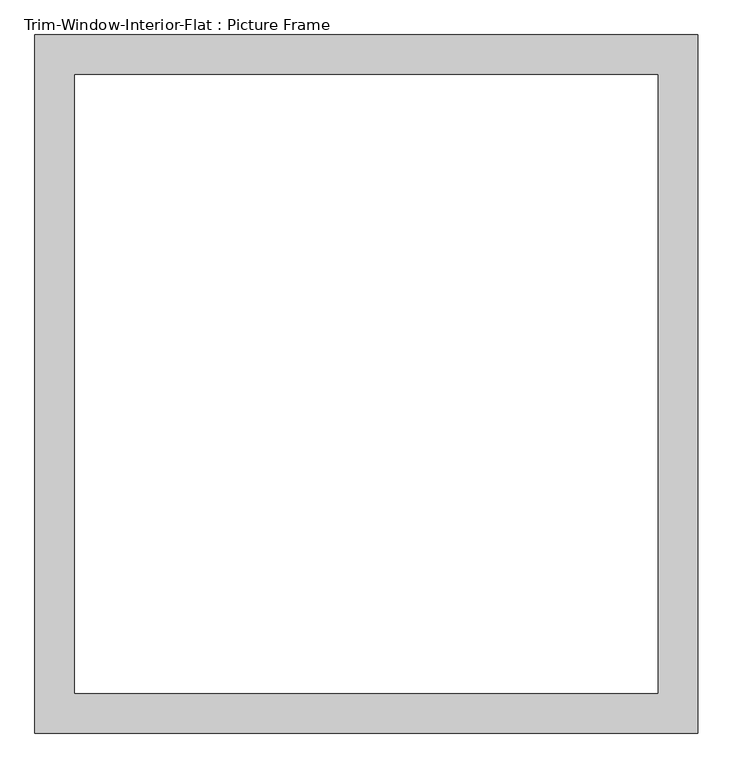
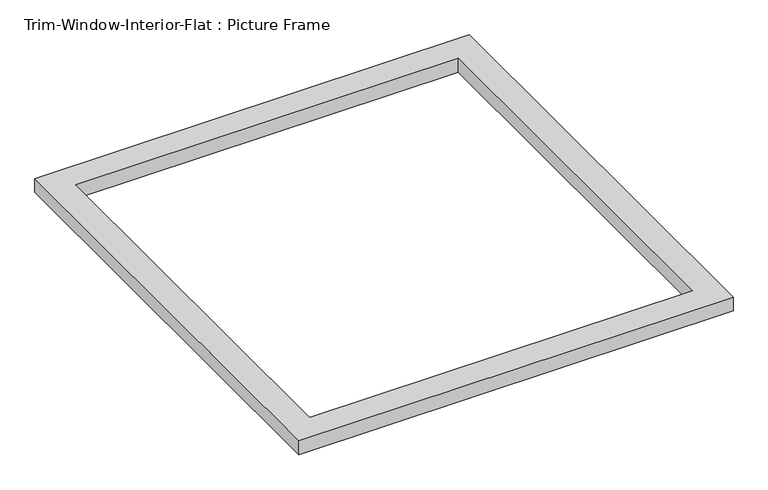
"""IFC4 building model written with IfcOpenShell, lengths in millimetres: proxy geometry, Trim-Window-Interior-Flat : Picture Frame."""

import ifcopenshell
import ifcopenshell.guid

model = None  # the IFC model being written
_history = None  # IfcOwnerHistory: only IFC2X3 demands one
_inside = {}  # id of a spatial element -> (the spatial element, [elements in it])
_under = {}  # id of a project, library or spatial element -> (it, [spatial elements below it])
_declared = {}  # id of a project -> (the project, [libraries it declares])
_typed = {}  # id of a type object -> (the type object, [elements of that type])
_made_of = {}  # id of a material, layer set ... -> (it, [elements and type objects made of it])


def new_model(schema):
    """Start an empty IFC model of exactly this schema.

    Asked for "IFC4X3", IfcOpenShell would pick the latest addendum, in which some entities
    have other attributes; the version numbers below select the first issue.
    IFC2X3 requires an IfcOwnerHistory on every rooted entity: one is made here for all.
    """
    global model, _history
    if schema == "IFC4X3":
        model = ifcopenshell.file(schema_version=(4, 3, 0, 0))
    else:
        model = ifcopenshell.file(schema=schema)
    _inside.clear()
    _under.clear()
    _declared.clear()
    _typed.clear()
    _made_of.clear()
    _history = None
    if model.schema == "IFC2X3":
        org = make("IfcOrganization", Name="unknown")
        user = make(
            "IfcPersonAndOrganization",
            ThePerson=make("IfcPerson", FamilyName="unknown"),
            TheOrganization=org,
        )
        app = make(
            "IfcApplication",
            ApplicationDeveloper=org,
            Version="unknown",
            ApplicationFullName="unknown",
            ApplicationIdentifier="unknown",
        )
        _history = make(
            "IfcOwnerHistory",
            OwningUser=user,
            OwningApplication=app,
            ChangeAction="ADDED",
            CreationDate=0,
        )
    return model


def make(cls, **values):
    """One entity of the class cls with the attributes given. An attribute that is None is left unset."""
    return model.create_entity(
        cls, **{name: value for name, value in values.items() if value is not None}
    )


def rooted(cls, **values):
    """An entity with a GlobalId (a new one), such as an element, a storey or a relation."""
    return make(cls, GlobalId=ifcopenshell.guid.new(), OwnerHistory=_history, **values)


def si_unit(unit_type, name, prefix=None):
    """IfcSIUnit, for example si_unit("LENGTHUNIT", "METRE", prefix="MILLI")."""
    return make("IfcSIUnit", UnitType=unit_type, Prefix=prefix, Name=name)


def assignment(units):
    """IfcUnitAssignment: the units of a project."""
    return None if units is None else make("IfcUnitAssignment", Units=units)


def point(xyz):
    """IfcCartesianPoint."""
    return None if xyz is None else make("IfcCartesianPoint", Coordinates=xyz)


def direction(xyz):
    """IfcDirection."""
    return None if xyz is None else make("IfcDirection", DirectionRatios=xyz)


def frame(location, z_axis=None, x_axis=None):
    """IfcAxis2Placement3D, a coordinate frame: its origin and axes. An axis left out is left unset."""
    return make(
        "IfcAxis2Placement3D",
        Location=point(location),
        Axis=direction(z_axis),
        RefDirection=direction(x_axis),
    )


def origin():
    """The frame at (0, 0, 0) with its axes left unset."""
    return frame((0.0, 0.0, 0.0))


def origin_with_axes():
    """The frame at (0, 0, 0) with the z axis (0, 0, 1) and the x axis (1, 0, 0) written out."""
    return frame((0.0, 0.0, 0.0), z_axis=(0.0, 0.0, 1.0), x_axis=(1.0, 0.0, 0.0))


def place(relative_to, where):
    """IfcLocalPlacement: puts the frame where relative to a parent placement (None: the world)."""
    return make(
        "IfcLocalPlacement", PlacementRelTo=relative_to, RelativePlacement=where
    )


def context(
    kind, dimensions, precision=None, world=None, true_north=None, identifier=None
):
    """IfcGeometricRepresentationContext, for example the 3D "Model" context."""
    return make(
        "IfcGeometricRepresentationContext",
        ContextIdentifier=identifier,
        ContextType=kind,
        CoordinateSpaceDimension=dimensions,
        Precision=precision,
        WorldCoordinateSystem=world,
        TrueNorth=true_north,
    )


def project(units=None, contexts=None):
    """IfcProject with its units and contexts."""
    return rooted(
        "IfcProject",
        Name="project",
        RepresentationContexts=contexts,
        UnitsInContext=assignment(units),
    )


def spatial(cls, under=None, at=None, **own):
    """A site, building, storey or space (cls), placed at a placement, below another one or the project."""
    s = rooted(cls, ObjectPlacement=at, **own)
    if under is not None:
        _under.setdefault(under.id(), (under, []))[1].append(s)
    return s


def polyline(points):
    """IfcPolyline through the points."""
    return make("IfcPolyline", Points=[point(p) for p in points])


def outline(outer, holes=None, kind="AREA"):
    """IfcArbitraryClosedProfileDef: a profile drawn as a closed curve; with holes, ...WithVoids."""
    if holes is None:
        return make("IfcArbitraryClosedProfileDef", ProfileType=kind, OuterCurve=outer)
    return make(
        "IfcArbitraryProfileDefWithVoids",
        ProfileType=kind,
        OuterCurve=outer,
        InnerCurves=holes,
    )


def extrude(swept, where, along, depth):
    """IfcExtrudedAreaSolid: the profile swept, set in the frame where, extruded along a direction by depth."""
    return make(
        "IfcExtrudedAreaSolid",
        SweptArea=swept,
        Position=where,
        ExtrudedDirection=direction(along),
        Depth=depth,
    )


def shape(context_of_items, identifier, shape_type, items):
    """IfcShapeRepresentation: the items that make up one representation, for example the "Body"."""
    return make(
        "IfcShapeRepresentation",
        ContextOfItems=context_of_items,
        RepresentationIdentifier=identifier,
        RepresentationType=shape_type,
        Items=items,
    )


def source(mapping_origin, context_of_items, identifier, shape_type, items):
    """IfcRepresentationMap: a shape defined once, which mapped items show again and again."""
    return make(
        "IfcRepresentationMap",
        MappingOrigin=mapping_origin,
        MappedRepresentation=shape(context_of_items, identifier, shape_type, items),
    )


def transform(
    local_origin,
    x_axis=None,
    y_axis=None,
    z_axis=None,
    scale=None,
    scale2=None,
    scale3=None,
    uniform=True,
):
    """IfcCartesianTransformationOperator3D, or its non-uniform kind. x_axis, y_axis, z_axis: its Axis1, 2, 3."""
    if uniform:
        return make(
            "IfcCartesianTransformationOperator3D",
            Axis1=direction(x_axis),
            Axis2=direction(y_axis),
            LocalOrigin=point(local_origin),
            Scale=scale,
            Axis3=direction(z_axis),
        )
    return make(
        "IfcCartesianTransformationOperator3DnonUniform",
        Axis1=direction(x_axis),
        Axis2=direction(y_axis),
        LocalOrigin=point(local_origin),
        Scale=scale,
        Axis3=direction(z_axis),
        Scale2=scale2,
        Scale3=scale3,
    )


def mapped(mapping_source, mapping_target):
    """IfcMappedItem: shows the shape of a source again, moved by a transform."""
    return make(
        "IfcMappedItem", MappingSource=mapping_source, MappingTarget=mapping_target
    )


def made_of(thing, what):
    """Note that an element or type object is made of a material, layer set ...; save() writes the relation."""
    if what is not None:
        _made_of.setdefault(what.id(), (what, []))[1].append(thing)
    return thing


def element(
    cls,
    number,
    at=None,
    inside=None,
    cuts=None,
    type_object=None,
    material=None,
    context=None,
    identifier="Body",
    shape_type=None,
    held_by="IfcProductDefinitionShape",
    body=None,
    shapes=None,
    **own,
):
    """One element of the class cls, such as IfcWall. Its Tag is "e" and its number.

    at: its placement. inside: the storey or other place that contains it. cuts: it is an
    opening in that element (IfcRelVoidsElement). A single representation is given by context,
    identifier, shape_type and body (its items); several are given by shapes. held_by: the class
    of the entity that holds the representations. save() writes the other relations.
    """
    e = rooted(cls, Tag="e%d" % number, ObjectPlacement=at, **own)
    if body is not None:
        shapes = [shape(context, identifier, shape_type, body)]
    if shapes is not None:
        e.Representation = make(held_by, Representations=shapes)
    if inside is not None:
        _inside.setdefault(inside.id(), (inside, []))[1].append(e)
    if cuts is not None:
        rooted(
            "IfcRelVoidsElement", RelatingBuildingElement=cuts, RelatedOpeningElement=e
        )
    if type_object is not None:
        _typed.setdefault(type_object.id(), (type_object, []))[1].append(e)
    return made_of(e, material)


def aggregate(whole, parts):
    """IfcRelAggregates: a whole, such as a stair, and the parts it consists of."""
    return rooted("IfcRelAggregates", RelatingObject=whole, RelatedObjects=parts)


def save(model, path):
    """Write the relations noted so far, then the file.

    IfcRelAggregates (storeys below a building ...), IfcRelContainedInSpatialStructure (elements
    in a storey), IfcRelDefinesByType, IfcRelAssociatesMaterial and IfcRelDeclares: one each for
    every whole, place, type object, material and project.
    """
    for whole, parts in _under.values():
        aggregate(whole, parts)
    for where, things in _inside.values():
        rooted(
            "IfcRelContainedInSpatialStructure",
            RelatedElements=things,
            RelatingStructure=where,
        )
    for kind, things in _typed.values():
        rooted("IfcRelDefinesByType", RelatedObjects=things, RelatingType=kind)
    for what, things in _made_of.values():
        rooted("IfcRelAssociatesMaterial", RelatedObjects=things, RelatingMaterial=what)
    for by, libraries in _declared.values():
        rooted("IfcRelDeclares", RelatingContext=by, RelatedDefinitions=libraries)
    model.write(path)


def trim_window_interior_flat_picture_frame_51c85655(model_context):
    return source(origin(), model_context, "Body", "SweptSolid", [
        extrude(outline(polyline([(476.25, 44.45), (476.25, -958.85), (-476.25, -958.85), (-476.25, 44.45), (476.25, 44.45)]), holes=[polyline([(419.1, -12.7), (-419.1, -12.7), (-419.1, -901.7), (419.1, -901.7), (419.1, -12.7)])]), origin_with_axes(), (0.0, 0.0, 1.0), 31.75),
    ])


if __name__ == "__main__":
    model = new_model("IFC4")
    model_context = context("Model", 3, world=origin())
    ifc_project = project(units=[si_unit("LENGTHUNIT", "METRE", prefix="MILLI")], contexts=[model_context])
    site = spatial("IfcSite", under=ifc_project)
    building = spatial("IfcBuilding", under=site)
    placement = place(None, origin())
    trim_window_interior_flat_picture_frame_shape = trim_window_interior_flat_picture_frame_51c85655(model_context)
    element("IfcBuildingElementProxy", 1, Name="Trim-Window-Interior-Flat : Picture Frame", ObjectType="Trim-Window-Interior-Flat : Picture Frame", at=placement, inside=building, context=model_context, shape_type="MappedRepresentation", body=[
        mapped(trim_window_interior_flat_picture_frame_shape, transform((0.0, 0.0, 0.0), x_axis=(1.0, 0.0, 0.0), y_axis=(0.0, 1.0, 0.0), z_axis=(0.0, 0.0, 1.0))),
    ])
    save(model, "model.ifc")

# Revit data of these elements
# Type "Trim-Window-Interior-Flat : Picture Frame"
#   Trim Thickness_Picture Frame = 0' - 1 1/4"
#   Trim Width = 0' - 2 1/4"
#   Trim Thickness_with Sill = 0' - 0 3/4"
#   Sill Thickness = 0' - 1 1/4"
#   Opening Width [instance default] = 2' - 0"
#   Opening Height [instance default] = 3' - 0"
#   Default Elevation = 4' - 0"
#   Sill = no
#   Picture Frame = yes
#   Trim Material [instance default] = none
# Element 1 (IfcBuildingElementProxy, "Trim-Window-Interior-Flat : Picture Frame")
#   Opening Width = 2' - 10"
#   Trim Material = Wood - Stained
#   Materials on its faces: "Wood - Stained"
# Materials
#   "Wood - Stained": class "Wood", colour RGB 224 178 126, transparency 0, Cost = 0
